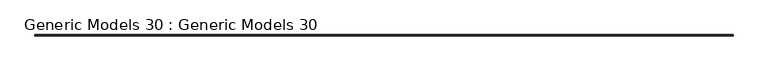
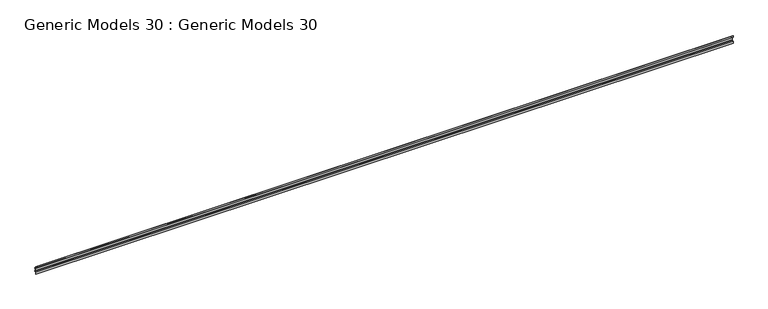
"""IFC4 building model written with IfcOpenShell, lengths in millimetres: proxy geometry, Generic Models 30 : Generic Models 30."""

from ifc_helpers import new_model, si_unit, point, frame, frame_2d, origin, place, context, project, spatial, polyline, circle_curve, trimmed, segment, composite_curve, outline, extrude, source, transform, mapped, element, save


def generic_models_30_generic_models_30_9ec8b5c7(model_context):
    return source(origin(), model_context, "Body", "SweptSolid", [
        extrude(outline(composite_curve([segment(polyline([(40961.0137657, 269410.6246691), (40970.2579, 269408.5857718)]), True, "CONTINUOUS"), segment(trimmed(circle_curve(frame_2d((40969.7450157, 269406.2604114)), 2.38125), [point((40970.2579, 269408.5857718))], [point((40971.3325157, 269404.4855324))], False, "CARTESIAN"), True, "CONTINUOUS"), segment(trimmed(circle_curve(frame_2d((40972.9200157, 269402.7106535)), 2.38125), [point((40971.3325157, 269404.4855324))], [point((40970.5387657, 269402.7106535))], True, "CARTESIAN"), True, "CONTINUOUS"), segment(polyline([(40970.5387657, 269402.7106535), (40970.5387657, 269382.0893465)]), True, "CONTINUOUS"), segment(trimmed(circle_curve(frame_2d((40972.9200157, 269382.0893465)), 2.38125), [point((40970.5387657, 269382.0893465))], [point((40971.3325157, 269380.3144676))], True, "CARTESIAN"), True, "CONTINUOUS"), segment(trimmed(circle_curve(frame_2d((40969.7450157, 269378.5395886)), 2.38125), [point((40971.3325157, 269380.3144676))], [point((40970.2579, 269376.2142282))], False, "CARTESIAN"), True, "CONTINUOUS"), segment(polyline([(40970.2579, 269376.2142282), (40961.0137657, 269374.1753309), (40961.0137657, 269360.65), (40959.4262657, 269360.65), (40959.4262657, 269375.4508453), (40969.9159772, 269377.7644685)]), True, "CONTINUOUS"), segment(trimmed(circle_curve(frame_2d((40969.7450157, 269378.5395886)), 0.79375), [point((40969.9159772, 269377.7644685))], [point((40970.2741824, 269379.1312149))], True, "CARTESIAN"), True, "CONTINUOUS"), segment(trimmed(circle_curve(frame_2d((40972.9200157, 269382.0893465)), 3.96875), [point((40970.2741824, 269379.1312149))], [point((40968.9512657, 269382.0893465))], False, "CARTESIAN"), True, "CONTINUOUS"), segment(polyline([(40968.9512657, 269382.0893465), (40968.9512657, 269402.7106535)]), True, "CONTINUOUS"), segment(trimmed(circle_curve(frame_2d((40972.9200157, 269402.7106535)), 3.96875), [point((40968.9512657, 269402.7106535))], [point((40970.2741824, 269405.6687851))], False, "CARTESIAN"), True, "CONTINUOUS"), segment(trimmed(circle_curve(frame_2d((40969.7450157, 269406.2604114)), 0.79375), [point((40970.2741824, 269405.6687851))], [point((40969.9159772, 269407.0355315))], True, "CARTESIAN"), True, "CONTINUOUS"), segment(polyline([(40969.9159772, 269407.0355315), (40959.4262657, 269409.3491547), (40959.4262657, 269424.15), (40961.0137657, 269424.15), (40961.0137657, 269410.6246691)]), True, "CONTINUOUS")], self_intersect=False)), frame((26427.4962986, 0.0, 0.0), z_axis=(1.0, 0.0, 0.0), x_axis=(0.0, 1.0, 0.0)), (0.0, 0.0, 1.0), 5733.6627792),
    ])


if __name__ == "__main__":
    model = new_model("IFC4")
    model_context = context("Model", 3, world=origin())
    ifc_project = project(units=[si_unit("LENGTHUNIT", "METRE", prefix="MILLI")], contexts=[model_context])
    site = spatial("IfcSite", under=ifc_project)
    building = spatial("IfcBuilding", under=site)
    placement = place(None, origin())
    generic_models_30_generic_models_30_shape = generic_models_30_generic_models_30_9ec8b5c7(model_context)
    element("IfcBuildingElementProxy", 1, Name="Generic Models 30 : Generic Models 30", ObjectType="Generic Models 30 : Generic Models 30", at=placement, inside=building, context=model_context, shape_type="MappedRepresentation", body=[
        mapped(generic_models_30_generic_models_30_shape, transform((0.0, 0.0, 0.0), x_axis=(1.0, 0.0, 0.0), y_axis=(0.0, 1.0, 0.0), z_axis=(0.0, 0.0, 1.0))),
    ])
    save(model, "model.ifc")

# Revit data of these elements
# Element 1 (IfcBuildingElementProxy, "Generic Models 30 : Generic Models 30")
#   Materials on its faces: "1/2\" DEEP GALV. HORTZ. HAT CHANNEL @ XX O.C."
# Materials
#   "1/2\" DEEP GALV. HORTZ. HAT CHANNEL @ XX O.C.": class "Generic", colour RGB 212 212 212, transparency 0, Cost = 0
